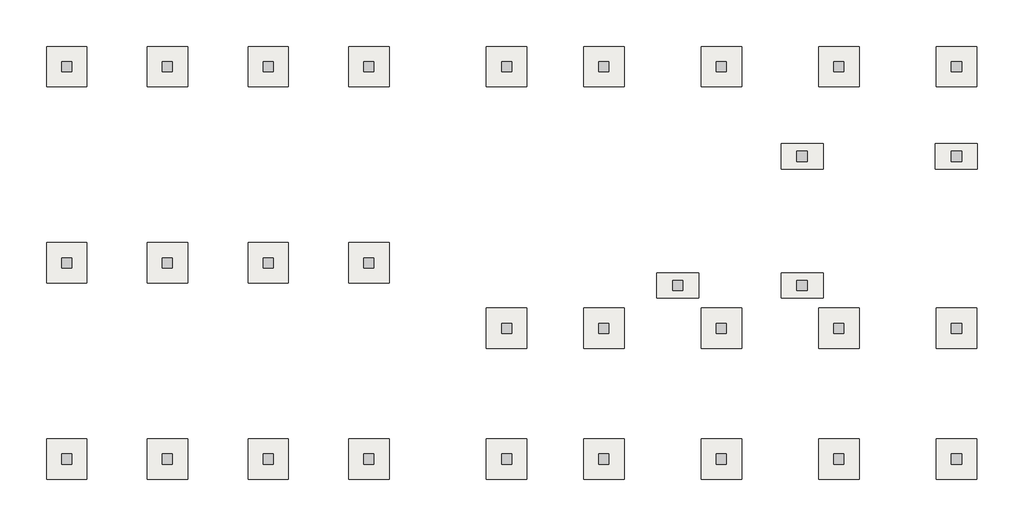
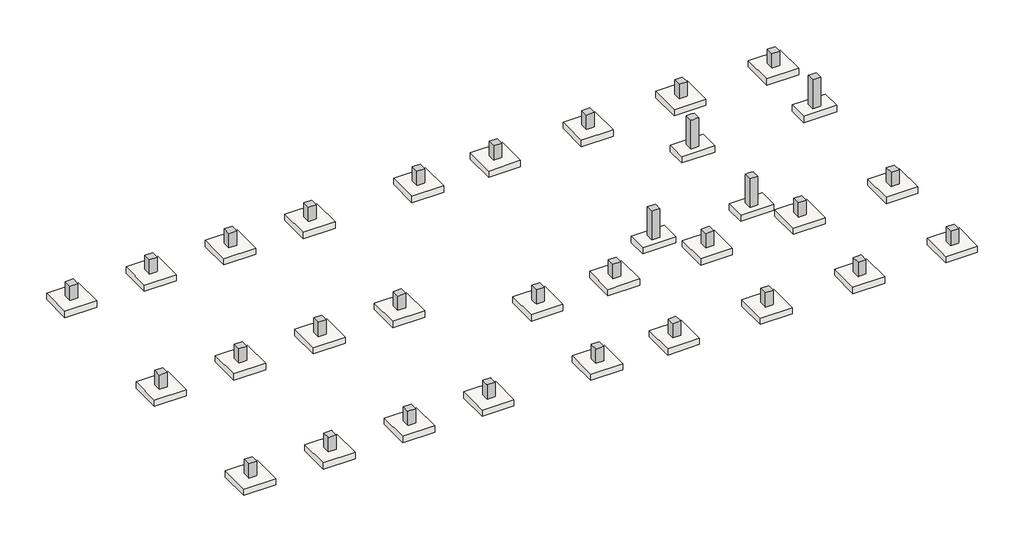
# Not in any storey: 31 columns, 31 slabs.
"""IFC4 building model written with IfcOpenShell, lengths in millimetres."""

from ifc_helpers import new_model, si_unit, frame, origin, place, context, project, spatial, polyline, outline, extrude, faceted_brep, element, save

model = new_model("IFC4")

# Units and contexts
model_context = context("Model", 3, world=origin())
ifc_project = project(units=[si_unit("LENGTHUNIT", "METRE", prefix="MILLI")], contexts=[model_context])

# Site, building
site = spatial("IfcSite", under=ifc_project)
building = spatial("IfcBuilding", under=site)

# Columns
placement = place(None, origin())
element("IfcColumn", 1, ObjectType="RC_Column_Rectangular : H_SC_ACC_UG PED_W600xL600", at=placement, inside=building, context=model_context, shape_type="SweptSolid", body=[
    extrude(outline(polyline([(224.7, 12616.5208589), (224.7, 12016.5208589), (-375.3, 12016.5208589), (-375.3, 12616.5208589), (224.7, 12616.5208589)])), frame((0.0, 0.0, -1150.0), z_axis=(0.0, 0.0, 1.0), x_axis=(1.0, 0.0, 0.0)), (0.0, 0.0, 1.0), 1150.0),
])
element("IfcColumn", 2, ObjectType="RC_Column_Rectangular : H_SC_ACC_UG PED_W600xL600", at=placement, inside=building, context=model_context, shape_type="SweptSolid", body=[
    extrude(outline(polyline([(6224.7, 12616.5208589), (6224.7, 12016.5208589), (5624.7, 12016.5208589), (5624.7, 12616.5208589), (6224.7, 12616.5208589)])), frame((0.0, 0.0, -1150.0), z_axis=(0.0, 0.0, 1.0), x_axis=(1.0, 0.0, 0.0)), (0.0, 0.0, 1.0), 1150.0),
])
element("IfcColumn", 3, ObjectType="RC_Column_Rectangular : H_SC_ACC_UG PED_W600xL600", at=placement, inside=building, context=model_context, shape_type="SweptSolid", body=[
    extrude(outline(polyline([(12224.7, 12616.5208589), (12224.7, 12016.5208589), (11624.7, 12016.5208589), (11624.7, 12616.5208589), (12224.7, 12616.5208589)])), frame((0.0, 0.0, -1150.0), z_axis=(0.0, 0.0, 1.0), x_axis=(1.0, 0.0, 0.0)), (0.0, 0.0, 1.0), 1150.0),
])
element("IfcColumn", 4, ObjectType="RC_Column_Rectangular : H_SC_ACC_UG PED_W600xL600", at=placement, inside=building, context=model_context, shape_type="SweptSolid", body=[
    extrude(outline(polyline([(18224.7, 12616.5208589), (18224.7, 12016.5208589), (17624.7, 12016.5208589), (17624.7, 12616.5208589), (18224.7, 12616.5208589)])), frame((0.0, 0.0, -1150.0), z_axis=(0.0, 0.0, 1.0), x_axis=(1.0, 0.0, 0.0)), (0.0, 0.0, 1.0), 1150.0),
])
element("IfcColumn", 5, ObjectType="RC_Column_Rectangular : H_SC_ACC_UG PED_W600xL600", at=placement, inside=building, context=model_context, shape_type="SweptSolid", body=[
    extrude(outline(polyline([(224.7, 24316.5208589), (224.7, 23716.5208589), (-375.3, 23716.5208589), (-375.3, 24316.5208589), (224.7, 24316.5208589)])), frame((0.0, 0.0, -1150.0), z_axis=(0.0, 0.0, 1.0), x_axis=(1.0, 0.0, 0.0)), (0.0, 0.0, 1.0), 1150.0),
])
element("IfcColumn", 6, ObjectType="RC_Column_Rectangular : H_SC_ACC_UG PED_W600xL600", at=placement, inside=building, context=model_context, shape_type="SweptSolid", body=[
    extrude(outline(polyline([(6224.7, 24316.5208589), (6224.7, 23716.5208589), (5624.7, 23716.5208589), (5624.7, 24316.5208589), (6224.7, 24316.5208589)])), frame((0.0, 0.0, -1150.0), z_axis=(0.0, 0.0, 1.0), x_axis=(1.0, 0.0, 0.0)), (0.0, 0.0, 1.0), 1150.0),
])
element("IfcColumn", 7, ObjectType="RC_Column_Rectangular : H_SC_ACC_UG PED_W600xL600", at=placement, inside=building, context=model_context, shape_type="SweptSolid", body=[
    extrude(outline(polyline([(12224.7, 24316.5208589), (12224.7, 23716.5208589), (11624.7, 23716.5208589), (11624.7, 24316.5208589), (12224.7, 24316.5208589)])), frame((0.0, 0.0, -1150.0), z_axis=(0.0, 0.0, 1.0), x_axis=(1.0, 0.0, 0.0)), (0.0, 0.0, 1.0), 1150.0),
])
element("IfcColumn", 8, ObjectType="RC_Column_Rectangular : H_SC_ACC_UG PED_W600xL600", at=placement, inside=building, context=model_context, shape_type="SweptSolid", body=[
    extrude(outline(polyline([(18224.7, 24316.5208589), (18224.7, 23716.5208589), (17624.7, 23716.5208589), (17624.7, 24316.5208589), (18224.7, 24316.5208589)])), frame((0.0, 0.0, -1150.0), z_axis=(0.0, 0.0, 1.0), x_axis=(1.0, 0.0, 0.0)), (0.0, 0.0, 1.0), 1150.0),
])
element("IfcColumn", 9, ObjectType="RC_Column_Rectangular : H_SC_ACC_UG PED_W600xL600", at=placement, inside=building, context=model_context, shape_type="SweptSolid", body=[
    extrude(outline(polyline([(26424.7, 24316.5208589), (26424.7, 23716.5208589), (25824.7, 23716.5208589), (25824.7, 24316.5208589), (26424.7, 24316.5208589)])), frame((0.0, 0.0, -1150.0), z_axis=(0.0, 0.0, 1.0), x_axis=(1.0, 0.0, 0.0)), (0.0, 0.0, 1.0), 1150.0),
])
element("IfcColumn", 10, ObjectType="RC_Column_Rectangular : H_SC_ACC_UG PED_W600xL600", at=placement, inside=building, context=model_context, shape_type="SweptSolid", body=[
    extrude(outline(polyline([(32224.7, 24316.5208589), (32224.7, 23716.5208589), (31624.7, 23716.5208589), (31624.7, 24316.5208589), (32224.7, 24316.5208589)])), frame((0.0, 0.0, -1150.0), z_axis=(0.0, 0.0, 1.0), x_axis=(1.0, 0.0, 0.0)), (0.0, 0.0, 1.0), 1150.0),
])
element("IfcColumn", 11, ObjectType="RC_Column_Rectangular : H_SC_ACC_UG PED_W600xL600", at=placement, inside=building, context=model_context, shape_type="SweptSolid", body=[
    extrude(outline(polyline([(39224.7, 24316.5208589), (39224.7, 23716.5208589), (38624.7, 23716.5208589), (38624.7, 24316.5208589), (39224.7, 24316.5208589)])), frame((0.0, 0.0, -1150.0), z_axis=(0.0, 0.0, 1.0), x_axis=(1.0, 0.0, 0.0)), (0.0, 0.0, 1.0), 1150.0),
])
element("IfcColumn", 12, ObjectType="RC_Column_Rectangular : H_SC_ACC_UG PED_W600xL600", at=placement, inside=building, context=model_context, shape_type="SweptSolid", body=[
    extrude(outline(polyline([(46224.7, 24316.5208589), (46224.7, 23716.5208589), (45624.7, 23716.5208589), (45624.7, 24316.5208589), (46224.7, 24316.5208589)])), frame((0.0, 0.0, -1150.0), z_axis=(0.0, 0.0, 1.0), x_axis=(1.0, 0.0, 0.0)), (0.0, 0.0, 1.0), 1150.0),
])
element("IfcColumn", 13, ObjectType="RC_Column_Rectangular : H_SC_ACC_UG PED_W600xL600", at=placement, inside=building, context=model_context, shape_type="SweptSolid", body=[
    extrude(outline(polyline([(53224.7, 24316.5208589), (53224.7, 23716.5208589), (52624.7, 23716.5208589), (52624.7, 24316.5208589), (53224.7, 24316.5208589)])), frame((0.0, 0.0, -1150.0), z_axis=(0.0, 0.0, 1.0), x_axis=(1.0, 0.0, 0.0)), (0.0, 0.0, 1.0), 1150.0),
])
element("IfcColumn", 14, ObjectType="RC_Column_Rectangular : H_SC_ACC_UG PED_W600xL600", at=placement, inside=building, context=model_context, shape_type="SweptSolid", body=[
    extrude(outline(polyline([(26424.7, 8716.5208589), (26424.7, 8116.5208589), (25824.7, 8116.5208589), (25824.7, 8716.5208589), (26424.7, 8716.5208589)])), frame((0.0, 0.0, -1150.0), z_axis=(0.0, 0.0, 1.0), x_axis=(1.0, 0.0, 0.0)), (0.0, 0.0, 1.0), 1150.0),
])
element("IfcColumn", 15, ObjectType="RC_Column_Rectangular : H_SC_ACC_UG PED_W600xL600", at=placement, inside=building, context=model_context, shape_type="SweptSolid", body=[
    extrude(outline(polyline([(32224.7, 8716.5208589), (32224.7, 8116.5208589), (31624.7, 8116.5208589), (31624.7, 8716.5208589), (32224.7, 8716.5208589)])), frame((0.0, 0.0, -1150.0), z_axis=(0.0, 0.0, 1.0), x_axis=(1.0, 0.0, 0.0)), (0.0, 0.0, 1.0), 1150.0),
])
element("IfcColumn", 16, ObjectType="RC_Column_Rectangular : H_SC_ACC_UG PED_W600xL600", at=placement, inside=building, context=model_context, shape_type="SweptSolid", body=[
    extrude(outline(polyline([(39224.7, 8716.5208589), (39224.7, 8116.5208589), (38624.7, 8116.5208589), (38624.7, 8716.5208589), (39224.7, 8716.5208589)])), frame((0.0, 0.0, -1150.0), z_axis=(0.0, 0.0, 1.0), x_axis=(1.0, 0.0, 0.0)), (0.0, 0.0, 1.0), 1150.0),
])
element("IfcColumn", 17, ObjectType="RC_Column_Rectangular : H_SC_ACC_UG PED_W600xL600", at=placement, inside=building, context=model_context, shape_type="SweptSolid", body=[
    extrude(outline(polyline([(46224.7, 8716.5208589), (46224.7, 8116.5208589), (45624.7, 8116.5208589), (45624.7, 8716.5208589), (46224.7, 8716.5208589)])), frame((0.0, 0.0, -1150.0), z_axis=(0.0, 0.0, 1.0), x_axis=(1.0, 0.0, 0.0)), (0.0, 0.0, 1.0), 1150.0),
])
element("IfcColumn", 18, ObjectType="RC_Column_Rectangular : H_SC_ACC_UG PED_W600xL600", at=placement, inside=building, context=model_context, shape_type="SweptSolid", body=[
    extrude(outline(polyline([(53224.7, 8716.5208589), (53224.7, 8116.5208589), (52624.7, 8116.5208589), (52624.7, 8716.5208589), (53224.7, 8716.5208589)])), frame((0.0, 0.0, -1150.0), z_axis=(0.0, 0.0, 1.0), x_axis=(1.0, 0.0, 0.0)), (0.0, 0.0, 1.0), 1150.0),
])
element("IfcColumn", 19, ObjectType="RC_Column_Rectangular : H_SC_ACC_UG PED_W600xL600", at=placement, inside=building, context=model_context, shape_type="Brep", body=[
    faceted_brep([(224.7, 916.5208589, -1150.0), (224.7, 316.5208589, -1150.0), (-375.3, 316.5208589, -1150.0), (-375.3, 916.5208589, -1150.0), (224.7, 916.5208589, 0.0), (224.7, 816.5208589, 0.0), (224.7, 416.5208589, 0.0), (224.7, 316.5208589, 0.0), (-375.3, 316.5208589, 0.0), (-375.3, 916.5208589, 0.0), (-275.3, 916.5208589, 0.0), (124.7, 916.5208589, 0.0)], [[[0, 1, 2, 3]], [[1, 0, 4, 5, 6, 7]], [[2, 1, 7, 8]], [[3, 2, 8, 9]], [[0, 3, 9, 10, 11, 4]], [[7, 6, 5, 4, 11, 10, 9, 8]]]),
])
element("IfcColumn", 20, ObjectType="RC_Column_Rectangular : H_SC_ACC_UG PED_W600xL600", at=placement, inside=building, context=model_context, shape_type="Brep", body=[
    faceted_brep([(6224.7, 916.5208589, -1150.0), (6224.7, 316.5208589, -1150.0), (5624.7, 316.5208589, -1150.0), (5624.7, 916.5208589, -1150.0), (6224.7, 916.5208589, 0.0), (6224.7, 816.5208589, 0.0), (6224.7, 416.5208589, 0.0), (6224.7, 316.5208589, 0.0), (5624.7, 316.5208589, 0.0), (5624.7, 416.5208589, 0.0), (5624.7, 816.5208589, 0.0), (5624.7, 916.5208589, 0.0)], [[[0, 1, 2, 3]], [[1, 0, 4, 5, 6, 7]], [[2, 1, 7, 8]], [[3, 2, 8, 9, 10, 11]], [[0, 3, 11, 4]], [[7, 6, 5, 4, 11, 10, 9, 8]]]),
])
element("IfcColumn", 21, ObjectType="RC_Column_Rectangular : H_SC_ACC_UG PED_W600xL600", at=placement, inside=building, context=model_context, shape_type="Brep", body=[
    faceted_brep([(12224.7, 916.5208589, -1150.0), (12224.7, 316.5208589, -1150.0), (11624.7, 316.5208589, -1150.0), (11624.7, 916.5208589, -1150.0), (12224.7, 916.5208589, 0.0), (12224.7, 816.5208589, 0.0), (12224.7, 416.5208589, 0.0), (12224.7, 316.5208589, 0.0), (11624.7, 316.5208589, 0.0), (11624.7, 416.5208589, 0.0), (11624.7, 816.5208589, 0.0), (11624.7, 916.5208589, 0.0)], [[[0, 1, 2, 3]], [[1, 0, 4, 5, 6, 7]], [[2, 1, 7, 8]], [[3, 2, 8, 9, 10, 11]], [[0, 3, 11, 4]], [[7, 6, 5, 4, 11, 10, 9, 8]]]),
])
element("IfcColumn", 22, ObjectType="RC_Column_Rectangular : H_SC_ACC_UG PED_W600xL600", at=placement, inside=building, context=model_context, shape_type="Brep", body=[
    faceted_brep([(18224.7, 916.5208589, -1150.0), (18224.7, 316.5208589, -1150.0), (17624.7, 316.5208589, -1150.0), (17624.7, 916.5208589, -1150.0), (18224.7, 916.5208589, 0.0), (18224.7, 816.5208589, 0.0), (18224.7, 416.5208589, 0.0), (18224.7, 316.5208589, 0.0), (17624.7, 316.5208589, 0.0), (17624.7, 416.5208589, 0.0), (17624.7, 816.5208589, 0.0), (17624.7, 916.5208589, 0.0)], [[[0, 1, 2, 3]], [[1, 0, 4, 5, 6, 7]], [[2, 1, 7, 8]], [[3, 2, 8, 9, 10, 11]], [[0, 3, 11, 4]], [[7, 6, 5, 4, 11, 10, 9, 8]]]),
])
element("IfcColumn", 23, ObjectType="RC_Column_Rectangular : H_SC_ACC_UG PED_W600xL600", at=placement, inside=building, context=model_context, shape_type="Brep", body=[
    faceted_brep([(26424.7, 916.5208589, -1150.0), (26424.7, 316.5208589, -1150.0), (25824.7, 316.5208589, -1150.0), (25824.7, 916.5208589, -1150.0), (26424.7, 916.5208589, 0.0), (26424.7, 316.5208589, 0.0), (25824.7, 316.5208589, 0.0), (25824.7, 416.5208589, 0.0), (25824.7, 816.5208589, 0.0), (25824.7, 916.5208589, 0.0)], [[[0, 1, 2, 3]], [[1, 0, 4, 5]], [[2, 1, 5, 6]], [[3, 2, 6, 7, 8, 9]], [[0, 3, 9, 4]], [[5, 4, 9, 8, 7, 6]]]),
])
element("IfcColumn", 24, ObjectType="RC_Column_Rectangular : H_SC_ACC_UG PED_W600xL600", at=placement, inside=building, context=model_context, shape_type="SweptSolid", body=[
    extrude(outline(polyline([(32224.7, 916.5208589), (32224.7, 316.5208589), (31624.7, 316.5208589), (31624.7, 916.5208589), (32224.7, 916.5208589)])), frame((0.0, 0.0, -1150.0), z_axis=(0.0, 0.0, 1.0), x_axis=(1.0, 0.0, 0.0)), (0.0, 0.0, 1.0), 1150.0),
])
element("IfcColumn", 25, ObjectType="RC_Column_Rectangular : H_SC_ACC_UG PED_W600xL600", at=placement, inside=building, context=model_context, shape_type="SweptSolid", body=[
    extrude(outline(polyline([(39224.7, 916.5208589), (39224.7, 316.5208589), (38624.7, 316.5208589), (38624.7, 916.5208589), (39224.7, 916.5208589)])), frame((0.0, 0.0, -1150.0), z_axis=(0.0, 0.0, 1.0), x_axis=(1.0, 0.0, 0.0)), (0.0, 0.0, 1.0), 1150.0),
])
element("IfcColumn", 26, ObjectType="RC_Column_Rectangular : H_SC_ACC_UG PED_W600xL600", at=placement, inside=building, context=model_context, shape_type="SweptSolid", body=[
    extrude(outline(polyline([(46224.7, 916.5208589), (46224.7, 316.5208589), (45624.7, 316.5208589), (45624.7, 916.5208589), (46224.7, 916.5208589)])), frame((0.0, 0.0, -1150.0), z_axis=(0.0, 0.0, 1.0), x_axis=(1.0, 0.0, 0.0)), (0.0, 0.0, 1.0), 1150.0),
])
element("IfcColumn", 27, ObjectType="RC_Column_Rectangular : H_SC_ACC_UG PED_W600xL600", at=placement, inside=building, context=model_context, shape_type="SweptSolid", body=[
    extrude(outline(polyline([(53224.7, 916.5208589), (53224.7, 316.5208589), (52624.7, 316.5208589), (52624.7, 916.5208589), (53224.7, 916.5208589)])), frame((0.0, 0.0, -1150.0), z_axis=(0.0, 0.0, 1.0), x_axis=(1.0, 0.0, 0.0)), (0.0, 0.0, 1.0), 1150.0),
])
element("IfcColumn", 28, ObjectType="RC_Column_Rectangular : H_SC_ACC_UG PED_W600xL600", at=placement, inside=building, context=model_context, shape_type="Brep", body=[
    faceted_brep([(36624.7, 11266.5208589, -1150.0), (36624.7, 10666.5208589, -1150.0), (36024.7, 10666.5208589, -1150.0), (36024.7, 11266.5208589, -1150.0), (36624.7, 11266.5208589, 1150.0), (36624.7, 11083.5208589, 1150.0), (36624.7, 10849.5208589, 1150.0), (36624.7, 10666.5208589, 1150.0), (36624.7, 10666.5208589, 1000.0), (36624.7, 11266.5208589, 50.0), (36624.7, 11266.5208589, 200.0), (36324.7, 10666.5208589, 1150.0), (36024.7, 10666.5208589, 1150.0), (36024.7, 10666.5208589, 200.0), (36024.7, 10666.5208589, 50.0), (36024.7, 11266.5208589, 1150.0), (36024.7, 11266.5208589, 200.0), (36024.7, 11266.5208589, 50.0)], [[[0, 1, 2, 3]], [[4, 5, 6, 7, 8, 1, 0, 9, 10]], [[7, 11, 12, 13, 14, 2, 1, 8]], [[12, 15, 16, 17, 3, 2, 14, 13]], [[15, 4, 10, 9, 0, 3, 17, 16]], [[4, 15, 12, 11, 7, 6, 5]]]),
])
element("IfcColumn", 29, ObjectType="RC_Column_Rectangular : H_SC_ACC_UG PED_W600xL600", at=placement, inside=building, context=model_context, shape_type="Brep", body=[
    faceted_brep([(44024.7, 11266.5208589, -1150.0), (44024.7, 10666.5208589, -1150.0), (43424.7, 10666.5208589, -1150.0), (43424.7, 11266.5208589, -1150.0), (44024.7, 11266.5208589, 1150.0), (44024.7, 11083.5208589, 1150.0), (44024.7, 10849.5208589, 1150.0), (44024.7, 10666.5208589, 1150.0), (44024.7, 10666.5208589, 1000.0), (44024.7, 11266.5208589, 1000.0), (43424.7, 10666.5208589, 1150.0), (43424.7, 10666.5208589, 1000.0), (43424.7, 10849.5208589, 1150.0), (43424.7, 11083.5208589, 1150.0), (43424.7, 11266.5208589, 1150.0), (43424.7, 11266.5208589, 200.0), (43424.7, 11266.5208589, 50.0), (43607.7, 11266.5208589, 1150.0), (43841.7, 11266.5208589, 1150.0)], [[[0, 1, 2, 3]], [[4, 5, 6, 7, 8, 1, 0, 9]], [[7, 10, 11, 2, 1, 8]], [[10, 12, 13, 14, 15, 16, 3, 2, 11]], [[14, 17, 18, 4, 9, 0, 3, 16, 15]], [[4, 18, 17, 14, 13, 12, 10, 7, 6, 5]]]),
])
element("IfcColumn", 30, ObjectType="RC_Column_Rectangular : H_SC_ACC_UG PED_W600xL600", at=placement, inside=building, context=model_context, shape_type="Brep", body=[
    faceted_brep([(44024.7, 18966.5208589, -1150.0), (44024.7, 18366.5208589, -1150.0), (43424.7, 18366.5208589, -1150.0), (43424.7, 18966.5208589, -1150.0), (44024.7, 18966.5208589, 1150.0), (44024.7, 18366.5208589, 1150.0), (44024.7, 18366.5208589, 1000.0), (44024.7, 18966.5208589, 1000.0), (43841.7, 18366.5208589, 1150.0), (43607.7, 18366.5208589, 1150.0), (43424.7, 18366.5208589, 1150.0), (43424.7, 18366.5208589, 200.0), (43424.7, 18366.5208589, 50.0), (43424.7, 18966.5208589, 1150.0), (43424.7, 18966.5208589, 200.0), (43424.7, 18966.5208589, 50.0), (43607.7, 18966.5208589, 1150.0), (43841.7, 18966.5208589, 1150.0)], [[[0, 1, 2, 3]], [[4, 5, 6, 1, 0, 7]], [[5, 8, 9, 10, 11, 12, 2, 1, 6]], [[10, 13, 14, 15, 3, 2, 12, 11]], [[13, 16, 17, 4, 7, 0, 3, 15, 14]], [[4, 17, 16, 13, 10, 9, 8, 5]]]),
])
element("IfcColumn", 31, ObjectType="RC_Column_Rectangular : H_SC_ACC_UG PED_W600xL600", at=placement, inside=building, context=model_context, shape_type="Brep", body=[
    faceted_brep([(53224.7, 18966.5208589, -1150.0), (53224.7, 18366.5208589, -1150.0), (52624.7, 18366.5208589, -1150.0), (52624.7, 18966.5208589, -1150.0), (53224.7, 18966.5208589, 1150.0), (53224.7, 18366.5208589, 1150.0), (53224.7, 18366.5208589, 150.0), (53224.7, 18966.5208589, 150.0), (52794.7, 18366.5208589, 1150.0), (52624.7, 18366.5208589, 1150.0), (52624.7, 18366.5208589, 1000.0), (52624.7, 18966.5208589, 1150.0), (52624.7, 18966.5208589, 1000.0), (52794.7, 18966.5208589, 1150.0)], [[[0, 1, 2, 3]], [[4, 5, 6, 1, 0, 7]], [[5, 8, 9, 10, 2, 1, 6]], [[9, 11, 12, 3, 2, 10]], [[11, 13, 4, 7, 0, 3, 12]], [[4, 13, 11, 9, 8, 5]]]),
])

# Slabs
element("IfcSlab", 32, ObjectType="FT211-Footing-Rectangular_R1 : H_SF_ACF_W2400xL2400xT500_Bitumen", at=placement, inside=building, context=model_context, shape_type="SweptSolid", body=[
    extrude(outline(polyline([(1124.7, 13516.5208589), (1124.7, 11116.5208589), (-1275.3, 11116.5208589), (-1275.3, 13516.5208589), (1124.7, 13516.5208589)])), frame((0.0, 0.0, -1650.0), z_axis=(0.0, 0.0, 1.0), x_axis=(1.0, 0.0, 0.0)), (0.0, 0.0, 1.0), 500.0),
])
element("IfcSlab", 33, ObjectType="FT211-Footing-Rectangular_R1 : H_SF_ACF_W2400xL2400xT500_Bitumen", at=placement, inside=building, context=model_context, shape_type="SweptSolid", body=[
    extrude(outline(polyline([(7124.7, 13516.5208589), (7124.7, 11116.5208589), (4724.7, 11116.5208589), (4724.7, 13516.5208589), (7124.7, 13516.5208589)])), frame((0.0, 0.0, -1650.0), z_axis=(0.0, 0.0, 1.0), x_axis=(1.0, 0.0, 0.0)), (0.0, 0.0, 1.0), 500.0),
])
element("IfcSlab", 34, ObjectType="FT211-Footing-Rectangular_R1 : H_SF_ACF_W2400xL2400xT500_Bitumen", at=placement, inside=building, context=model_context, shape_type="SweptSolid", body=[
    extrude(outline(polyline([(13124.7, 13516.5208589), (13124.7, 11116.5208589), (10724.7, 11116.5208589), (10724.7, 13516.5208589), (13124.7, 13516.5208589)])), frame((0.0, 0.0, -1650.0), z_axis=(0.0, 0.0, 1.0), x_axis=(1.0, 0.0, 0.0)), (0.0, 0.0, 1.0), 500.0),
])
element("IfcSlab", 35, ObjectType="FT211-Footing-Rectangular_R1 : H_SF_ACF_W2400xL2400xT500_Bitumen", at=placement, inside=building, context=model_context, shape_type="SweptSolid", body=[
    extrude(outline(polyline([(19124.7, 13516.5208589), (19124.7, 11116.5208589), (16724.7, 11116.5208589), (16724.7, 13516.5208589), (19124.7, 13516.5208589)])), frame((0.0, 0.0, -1650.0), z_axis=(0.0, 0.0, 1.0), x_axis=(1.0, 0.0, 0.0)), (0.0, 0.0, 1.0), 500.0),
])
element("IfcSlab", 36, ObjectType="FT211-Footing-Rectangular_R1 : H_SF_ACF_W2400xL2400xT500_Bitumen", at=placement, inside=building, context=model_context, shape_type="SweptSolid", body=[
    extrude(outline(polyline([(1124.7, 25216.5208589), (1124.7, 22816.5208589), (-1275.3, 22816.5208589), (-1275.3, 25216.5208589), (1124.7, 25216.5208589)])), frame((0.0, 0.0, -1650.0), z_axis=(0.0, 0.0, 1.0), x_axis=(1.0, 0.0, 0.0)), (0.0, 0.0, 1.0), 500.0),
])
element("IfcSlab", 37, ObjectType="FT211-Footing-Rectangular_R1 : H_SF_ACF_W2400xL2400xT500_Bitumen", at=placement, inside=building, context=model_context, shape_type="SweptSolid", body=[
    extrude(outline(polyline([(7124.7, 25216.5208589), (7124.7, 22816.5208589), (4724.7, 22816.5208589), (4724.7, 25216.5208589), (7124.7, 25216.5208589)])), frame((0.0, 0.0, -1650.0), z_axis=(0.0, 0.0, 1.0), x_axis=(1.0, 0.0, 0.0)), (0.0, 0.0, 1.0), 500.0),
])
element("IfcSlab", 38, ObjectType="FT211-Footing-Rectangular_R1 : H_SF_ACF_W2400xL2400xT500_Bitumen", at=placement, inside=building, context=model_context, shape_type="SweptSolid", body=[
    extrude(outline(polyline([(13124.7, 25216.5208589), (13124.7, 22816.5208589), (10724.7, 22816.5208589), (10724.7, 25216.5208589), (13124.7, 25216.5208589)])), frame((0.0, 0.0, -1650.0), z_axis=(0.0, 0.0, 1.0), x_axis=(1.0, 0.0, 0.0)), (0.0, 0.0, 1.0), 500.0),
])
element("IfcSlab", 39, ObjectType="FT211-Footing-Rectangular_R1 : H_SF_ACF_W2400xL2400xT500_Bitumen", at=placement, inside=building, context=model_context, shape_type="SweptSolid", body=[
    extrude(outline(polyline([(19124.7, 25216.5208589), (19124.7, 22816.5208589), (16724.7, 22816.5208589), (16724.7, 25216.5208589), (19124.7, 25216.5208589)])), frame((0.0, 0.0, -1650.0), z_axis=(0.0, 0.0, 1.0), x_axis=(1.0, 0.0, 0.0)), (0.0, 0.0, 1.0), 500.0),
])
element("IfcSlab", 40, ObjectType="FT211-Footing-Rectangular_R1 : H_SF_ACF_W2400xL2400xT500_Bitumen", at=placement, inside=building, context=model_context, shape_type="SweptSolid", body=[
    extrude(outline(polyline([(27324.7, 25216.5208589), (27324.7, 22816.5208589), (24924.7, 22816.5208589), (24924.7, 25216.5208589), (27324.7, 25216.5208589)])), frame((0.0, 0.0, -1650.0), z_axis=(0.0, 0.0, 1.0), x_axis=(1.0, 0.0, 0.0)), (0.0, 0.0, 1.0), 500.0),
])
element("IfcSlab", 41, ObjectType="FT211-Footing-Rectangular_R1 : H_SF_ACF_W2400xL2400xT500_Bitumen", at=placement, inside=building, context=model_context, shape_type="SweptSolid", body=[
    extrude(outline(polyline([(33124.7, 25216.5208589), (33124.7, 22816.5208589), (30724.7, 22816.5208589), (30724.7, 25216.5208589), (33124.7, 25216.5208589)])), frame((0.0, 0.0, -1650.0), z_axis=(0.0, 0.0, 1.0), x_axis=(1.0, 0.0, 0.0)), (0.0, 0.0, 1.0), 500.0),
])
element("IfcSlab", 42, ObjectType="FT211-Footing-Rectangular_R1 : H_SF_ACF_W2400xL2400xT500_Bitumen", at=placement, inside=building, context=model_context, shape_type="SweptSolid", body=[
    extrude(outline(polyline([(40124.7, 25216.5208589), (40124.7, 22816.5208589), (37724.7, 22816.5208589), (37724.7, 25216.5208589), (40124.7, 25216.5208589)])), frame((0.0, 0.0, -1650.0), z_axis=(0.0, 0.0, 1.0), x_axis=(1.0, 0.0, 0.0)), (0.0, 0.0, 1.0), 500.0),
])
element("IfcSlab", 43, ObjectType="FT211-Footing-Rectangular_R1 : H_SF_ACF_W2400xL2400xT500_Bitumen", at=placement, inside=building, context=model_context, shape_type="SweptSolid", body=[
    extrude(outline(polyline([(47124.7, 25216.5208589), (47124.7, 22816.5208589), (44724.7, 22816.5208589), (44724.7, 25216.5208589), (47124.7, 25216.5208589)])), frame((0.0, 0.0, -1650.0), z_axis=(0.0, 0.0, 1.0), x_axis=(1.0, 0.0, 0.0)), (0.0, 0.0, 1.0), 500.0),
])
element("IfcSlab", 44, ObjectType="FT211-Footing-Rectangular_R1 : H_SF_ACF_W2400xL2400xT500_Bitumen", at=placement, inside=building, context=model_context, shape_type="SweptSolid", body=[
    extrude(outline(polyline([(54124.7, 25216.5208589), (54124.7, 22816.5208589), (51724.7, 22816.5208589), (51724.7, 25216.5208589), (54124.7, 25216.5208589)])), frame((0.0, 0.0, -1650.0), z_axis=(0.0, 0.0, 1.0), x_axis=(1.0, 0.0, 0.0)), (0.0, 0.0, 1.0), 500.0),
])
element("IfcSlab", 45, ObjectType="FT211-Footing-Rectangular_R1 : H_SF_ACF_W2400xL2400xT500_Bitumen", at=placement, inside=building, context=model_context, shape_type="SweptSolid", body=[
    extrude(outline(polyline([(27324.7, 9616.5208589), (27324.7, 7216.5208589), (24924.7, 7216.5208589), (24924.7, 9616.5208589), (27324.7, 9616.5208589)])), frame((0.0, 0.0, -1650.0), z_axis=(0.0, 0.0, 1.0), x_axis=(1.0, 0.0, 0.0)), (0.0, 0.0, 1.0), 500.0),
])
element("IfcSlab", 46, ObjectType="FT211-Footing-Rectangular_R1 : H_SF_ACF_W2400xL2400xT500_Bitumen", at=placement, inside=building, context=model_context, shape_type="SweptSolid", body=[
    extrude(outline(polyline([(33124.7, 9616.5208589), (33124.7, 7216.5208589), (30724.7, 7216.5208589), (30724.7, 9616.5208589), (33124.7, 9616.5208589)])), frame((0.0, 0.0, -1650.0), z_axis=(0.0, 0.0, 1.0), x_axis=(1.0, 0.0, 0.0)), (0.0, 0.0, 1.0), 500.0),
])
element("IfcSlab", 47, ObjectType="FT211-Footing-Rectangular_R1 : H_SF_ACF_W2400xL2400xT500_Bitumen", at=placement, inside=building, context=model_context, shape_type="SweptSolid", body=[
    extrude(outline(polyline([(40124.7, 9616.5208589), (40124.7, 7216.5208589), (37724.7, 7216.5208589), (37724.7, 9616.5208589), (40124.7, 9616.5208589)])), frame((0.0, 0.0, -1650.0), z_axis=(0.0, 0.0, 1.0), x_axis=(1.0, 0.0, 0.0)), (0.0, 0.0, 1.0), 500.0),
])
element("IfcSlab", 48, ObjectType="FT211-Footing-Rectangular_R1 : H_SF_ACF_W2400xL2400xT500_Bitumen", at=placement, inside=building, context=model_context, shape_type="SweptSolid", body=[
    extrude(outline(polyline([(47124.7, 9616.5208589), (47124.7, 7216.5208589), (44724.7, 7216.5208589), (44724.7, 9616.5208589), (47124.7, 9616.5208589)])), frame((0.0, 0.0, -1650.0), z_axis=(0.0, 0.0, 1.0), x_axis=(1.0, 0.0, 0.0)), (0.0, 0.0, 1.0), 500.0),
])
element("IfcSlab", 49, ObjectType="FT211-Footing-Rectangular_R1 : H_SF_ACF_W2400xL2400xT500_Bitumen", at=placement, inside=building, context=model_context, shape_type="SweptSolid", body=[
    extrude(outline(polyline([(54124.7, 9616.5208589), (54124.7, 7216.5208589), (51724.7, 7216.5208589), (51724.7, 9616.5208589), (54124.7, 9616.5208589)])), frame((0.0, 0.0, -1650.0), z_axis=(0.0, 0.0, 1.0), x_axis=(1.0, 0.0, 0.0)), (0.0, 0.0, 1.0), 500.0),
])
element("IfcSlab", 50, ObjectType="FT211-Footing-Rectangular_R1 : H_SF_ACF_W2400xL2400xT500_Bitumen", at=placement, inside=building, context=model_context, shape_type="SweptSolid", body=[
    extrude(outline(polyline([(1124.7, 1816.5208589), (1124.7, -583.4791411), (-1275.3, -583.4791411), (-1275.3, 1816.5208589), (1124.7, 1816.5208589)])), frame((0.0, 0.0, -1650.0), z_axis=(0.0, 0.0, 1.0), x_axis=(1.0, 0.0, 0.0)), (0.0, 0.0, 1.0), 500.0),
])
element("IfcSlab", 51, ObjectType="FT211-Footing-Rectangular_R1 : H_SF_ACF_W2400xL2400xT500_Bitumen", at=placement, inside=building, context=model_context, shape_type="SweptSolid", body=[
    extrude(outline(polyline([(7124.7, 1816.5208589), (7124.7, -583.4791411), (4724.7, -583.4791411), (4724.7, 1816.5208589), (7124.7, 1816.5208589)])), frame((0.0, 0.0, -1650.0), z_axis=(0.0, 0.0, 1.0), x_axis=(1.0, 0.0, 0.0)), (0.0, 0.0, 1.0), 500.0),
])
element("IfcSlab", 52, ObjectType="FT211-Footing-Rectangular_R1 : H_SF_ACF_W2400xL2400xT500_Bitumen", at=placement, inside=building, context=model_context, shape_type="SweptSolid", body=[
    extrude(outline(polyline([(13124.7, 1816.5208589), (13124.7, -583.4791411), (10724.7, -583.4791411), (10724.7, 1816.5208589), (13124.7, 1816.5208589)])), frame((0.0, 0.0, -1650.0), z_axis=(0.0, 0.0, 1.0), x_axis=(1.0, 0.0, 0.0)), (0.0, 0.0, 1.0), 500.0),
])
element("IfcSlab", 53, ObjectType="FT211-Footing-Rectangular_R1 : H_SF_ACF_W2400xL2400xT500_Bitumen", at=placement, inside=building, context=model_context, shape_type="SweptSolid", body=[
    extrude(outline(polyline([(19124.7, 1816.5208589), (19124.7, -583.4791411), (16724.7, -583.4791411), (16724.7, 1816.5208589), (19124.7, 1816.5208589)])), frame((0.0, 0.0, -1650.0), z_axis=(0.0, 0.0, 1.0), x_axis=(1.0, 0.0, 0.0)), (0.0, 0.0, 1.0), 500.0),
])
element("IfcSlab", 54, ObjectType="FT211-Footing-Rectangular_R1 : H_SF_ACF_W2400xL2400xT500_Bitumen", at=placement, inside=building, context=model_context, shape_type="SweptSolid", body=[
    extrude(outline(polyline([(27324.7, 1816.5208589), (27324.7, -583.4791411), (24924.7, -583.4791411), (24924.7, 1816.5208589), (27324.7, 1816.5208589)])), frame((0.0, 0.0, -1650.0), z_axis=(0.0, 0.0, 1.0), x_axis=(1.0, 0.0, 0.0)), (0.0, 0.0, 1.0), 500.0),
])
element("IfcSlab", 55, ObjectType="FT211-Footing-Rectangular_R1 : H_SF_ACF_W2400xL2400xT500_Bitumen", at=placement, inside=building, context=model_context, shape_type="SweptSolid", body=[
    extrude(outline(polyline([(33124.7, 1816.5208589), (33124.7, -583.4791411), (30724.7, -583.4791411), (30724.7, 1816.5208589), (33124.7, 1816.5208589)])), frame((0.0, 0.0, -1650.0), z_axis=(0.0, 0.0, 1.0), x_axis=(1.0, 0.0, 0.0)), (0.0, 0.0, 1.0), 500.0),
])
element("IfcSlab", 56, ObjectType="FT211-Footing-Rectangular_R1 : H_SF_ACF_W2400xL2400xT500_Bitumen", at=placement, inside=building, context=model_context, shape_type="SweptSolid", body=[
    extrude(outline(polyline([(40124.7, 1816.5208589), (40124.7, -583.4791411), (37724.7, -583.4791411), (37724.7, 1816.5208589), (40124.7, 1816.5208589)])), frame((0.0, 0.0, -1650.0), z_axis=(0.0, 0.0, 1.0), x_axis=(1.0, 0.0, 0.0)), (0.0, 0.0, 1.0), 500.0),
])
element("IfcSlab", 57, ObjectType="FT211-Footing-Rectangular_R1 : H_SF_ACF_W2400xL2400xT500_Bitumen", at=placement, inside=building, context=model_context, shape_type="SweptSolid", body=[
    extrude(outline(polyline([(47124.7, 1816.5208589), (47124.7, -583.4791411), (44724.7, -583.4791411), (44724.7, 1816.5208589), (47124.7, 1816.5208589)])), frame((0.0, 0.0, -1650.0), z_axis=(0.0, 0.0, 1.0), x_axis=(1.0, 0.0, 0.0)), (0.0, 0.0, 1.0), 500.0),
])
element("IfcSlab", 58, ObjectType="FT211-Footing-Rectangular_R1 : H_SF_ACF_W2400xL2400xT500_Bitumen", at=placement, inside=building, context=model_context, shape_type="SweptSolid", body=[
    extrude(outline(polyline([(54124.7, 1816.5208589), (54124.7, -583.4791411), (51724.7, -583.4791411), (51724.7, 1816.5208589), (54124.7, 1816.5208589)])), frame((0.0, 0.0, -1650.0), z_axis=(0.0, 0.0, 1.0), x_axis=(1.0, 0.0, 0.0)), (0.0, 0.0, 1.0), 500.0),
])
element("IfcSlab", 59, ObjectType="FT211-Footing-Rectangular_R1 : H_SF_ACF_W2500xL1500xT500_Bitumen", at=placement, inside=building, context=model_context, shape_type="SweptSolid", body=[
    extrude(outline(polyline([(37574.7, 11716.5208589), (37574.7, 10216.5208589), (35074.7, 10216.5208589), (35074.7, 11716.5208589), (37574.7, 11716.5208589)])), frame((0.0, 0.0, -1650.0), z_axis=(0.0, 0.0, 1.0), x_axis=(1.0, 0.0, 0.0)), (0.0, 0.0, 1.0), 500.0),
])
element("IfcSlab", 60, ObjectType="FT211-Footing-Rectangular_R1 : H_SF_ACF_W2500xL1500xT500_Bitumen", at=placement, inside=building, context=model_context, shape_type="SweptSolid", body=[
    extrude(outline(polyline([(44974.7, 11716.5208589), (44974.7, 10216.5208589), (42474.7, 10216.5208589), (42474.7, 11716.5208589), (44974.7, 11716.5208589)])), frame((0.0, 0.0, -1650.0), z_axis=(0.0, 0.0, 1.0), x_axis=(1.0, 0.0, 0.0)), (0.0, 0.0, 1.0), 500.0),
])
element("IfcSlab", 61, ObjectType="FT211-Footing-Rectangular_R1 : H_SF_ACF_W2500xL1500xT500_Bitumen", at=placement, inside=building, context=model_context, shape_type="SweptSolid", body=[
    extrude(outline(polyline([(44974.7, 19416.5208589), (44974.7, 17916.5208589), (42474.7, 17916.5208589), (42474.7, 19416.5208589), (44974.7, 19416.5208589)])), frame((0.0, 0.0, -1650.0), z_axis=(0.0, 0.0, 1.0), x_axis=(1.0, 0.0, 0.0)), (0.0, 0.0, 1.0), 500.0),
])
element("IfcSlab", 62, ObjectType="FT211-Footing-Rectangular_R1 : H_SF_ACF_W2500xL1500xT500_Bitumen", at=placement, inside=building, context=model_context, shape_type="SweptSolid", body=[
    extrude(outline(polyline([(54174.7, 19416.5208589), (54174.7, 17916.5208589), (51674.7, 17916.5208589), (51674.7, 19416.5208589), (54174.7, 19416.5208589)])), frame((0.0, 0.0, -1650.0), z_axis=(0.0, 0.0, 1.0), x_axis=(1.0, 0.0, 0.0)), (0.0, 0.0, 1.0), 500.0),
])

save(model, "model.ifc")

# Revit data of these elements
# Type "RC_Column_Rectangular : H_SC_ACC_UG PED_W600xL600"
#   Width = 600.000 mm
#   Length = 600.000 mm
#   hec_material3 [instance default] = none
#   hec_material2 [instance default] = none
#   hec_material1 [instance default] = none
#   Structural Material [instance default] = none
#   Description = (empty or 0)
# Type "FT211-Footing-Rectangular_R1 : H_SF_ACF_W2400xL2400xT500_Bitumen"
#   Top bar = "D25@300"
#   Description = "UG Shallow Foundation"
#   Bottom bar = "D20@300"
#   Width = 2400.000 mm
#   Length = 2400.000 mm
#   Foundation Thickness = 500.000 mm
#   Structural Material [instance default] = none
#   Assembly Code = ""
# Type "FT211-Footing-Rectangular_R1 : H_SF_ACF_W2500xL1500xT500_Bitumen"
#   Top bar = "D25@300"
#   Description = "UG Shallow Foundation"
#   Bottom bar = "D20@300"
#   Width = 2500.000 mm
#   Length = 1500.000 mm
#   Foundation Thickness = 500.000 mm
#   Structural Material [instance default] = none
#   Assembly Code = ""
# Elements 1, 2, 3, 4, 5, 6, 7, 8, 9, 10, 11, 12, 13, 14, 15, 16, 17, 18, 19, 20, 21, 22, 23, 24, 25, 26, 27, 28, 29, 30, 31 (IfcColumn, "RC_Column_Rectangular : H_SC_ACC_UG PED_W600xL600")
#   Comments = ""
#   hec_material3 = none
#   hec_material2 = none
#   hec_material1 = none
#   Structural Material = none
#   Phase Created = New Construction
# Elements 32, 33, 34, 35, 36, 37, 38, 39, 40, 41, 42, 43, 44, 45, 46, 47, 48, 49, 50, 51, 52, 53, 54, 55, 56, 57, 58 (IfcSlab, "FT211-Footing-Rectangular_R1 : H_SF_ACF_W2400xL2400xT500_Bitumen")
#   Comments = ""
#   Structural Material = none
#   Phase Created = New Construction
# Elements 59, 60, 61, 62 (IfcSlab, "FT211-Footing-Rectangular_R1 : H_SF_ACF_W2500xL1500xT500_Bitumen")
#   Comments = ""
#   Structural Material = none
#   Phase Created = New Construction
